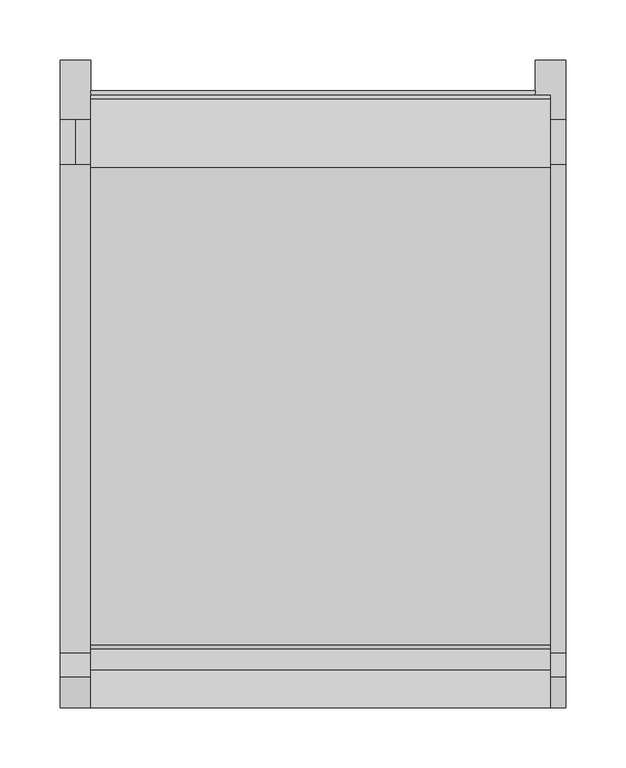
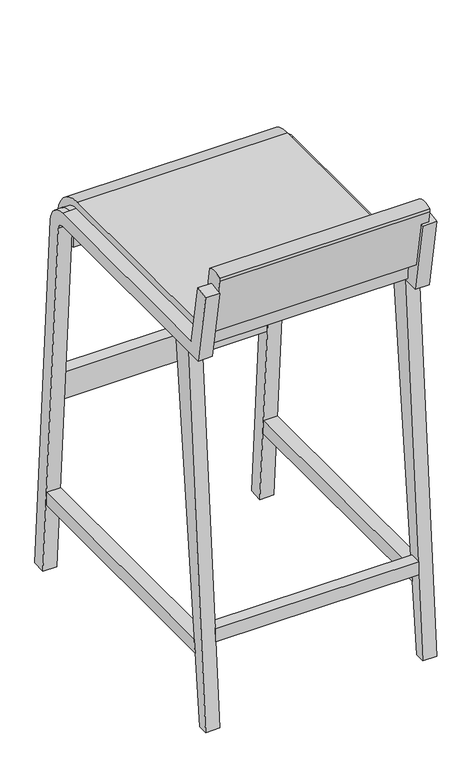
"""IFC4 building model written with IfcOpenShell, lengths in millimetres: furniture geometry, Bar_Stool_6722[1] : Bar_Stool_6722[1]."""

import ifcopenshell
import ifcopenshell.guid

model = None  # the IFC model being written
_history = None  # IfcOwnerHistory: only IFC2X3 demands one
_inside = {}  # id of a spatial element -> (the spatial element, [elements in it])
_under = {}  # id of a project, library or spatial element -> (it, [spatial elements below it])
_declared = {}  # id of a project -> (the project, [libraries it declares])
_typed = {}  # id of a type object -> (the type object, [elements of that type])
_made_of = {}  # id of a material, layer set ... -> (it, [elements and type objects made of it])


def new_model(schema):
    """Start an empty IFC model of exactly this schema.

    Asked for "IFC4X3", IfcOpenShell would pick the latest addendum, in which some entities
    have other attributes; the version numbers below select the first issue.
    IFC2X3 requires an IfcOwnerHistory on every rooted entity: one is made here for all.
    """
    global model, _history
    if schema == "IFC4X3":
        model = ifcopenshell.file(schema_version=(4, 3, 0, 0))
    else:
        model = ifcopenshell.file(schema=schema)
    _inside.clear()
    _under.clear()
    _declared.clear()
    _typed.clear()
    _made_of.clear()
    _history = None
    if model.schema == "IFC2X3":
        org = make("IfcOrganization", Name="unknown")
        user = make(
            "IfcPersonAndOrganization",
            ThePerson=make("IfcPerson", FamilyName="unknown"),
            TheOrganization=org,
        )
        app = make(
            "IfcApplication",
            ApplicationDeveloper=org,
            Version="unknown",
            ApplicationFullName="unknown",
            ApplicationIdentifier="unknown",
        )
        _history = make(
            "IfcOwnerHistory",
            OwningUser=user,
            OwningApplication=app,
            ChangeAction="ADDED",
            CreationDate=0,
        )
    return model


def make(cls, **values):
    """One entity of the class cls with the attributes given. An attribute that is None is left unset."""
    return model.create_entity(
        cls, **{name: value for name, value in values.items() if value is not None}
    )


def rooted(cls, **values):
    """An entity with a GlobalId (a new one), such as an element, a storey or a relation."""
    return make(cls, GlobalId=ifcopenshell.guid.new(), OwnerHistory=_history, **values)


def si_unit(unit_type, name, prefix=None):
    """IfcSIUnit, for example si_unit("LENGTHUNIT", "METRE", prefix="MILLI")."""
    return make("IfcSIUnit", UnitType=unit_type, Prefix=prefix, Name=name)


def assignment(units):
    """IfcUnitAssignment: the units of a project."""
    return None if units is None else make("IfcUnitAssignment", Units=units)


def point(xyz):
    """IfcCartesianPoint."""
    return None if xyz is None else make("IfcCartesianPoint", Coordinates=xyz)


def direction(xyz):
    """IfcDirection."""
    return None if xyz is None else make("IfcDirection", DirectionRatios=xyz)


def frame(location, z_axis=None, x_axis=None):
    """IfcAxis2Placement3D, a coordinate frame: its origin and axes. An axis left out is left unset."""
    return make(
        "IfcAxis2Placement3D",
        Location=point(location),
        Axis=direction(z_axis),
        RefDirection=direction(x_axis),
    )


def frame_2d(location, x_axis=None):
    """IfcAxis2Placement2D, a coordinate frame in the plane: its origin and x axis."""
    return make(
        "IfcAxis2Placement2D", Location=point(location), RefDirection=direction(x_axis)
    )


def origin():
    """The frame at (0, 0, 0) with its axes left unset."""
    return frame((0.0, 0.0, 0.0))


def place(relative_to, where):
    """IfcLocalPlacement: puts the frame where relative to a parent placement (None: the world)."""
    return make(
        "IfcLocalPlacement", PlacementRelTo=relative_to, RelativePlacement=where
    )


def context(
    kind, dimensions, precision=None, world=None, true_north=None, identifier=None
):
    """IfcGeometricRepresentationContext, for example the 3D "Model" context."""
    return make(
        "IfcGeometricRepresentationContext",
        ContextIdentifier=identifier,
        ContextType=kind,
        CoordinateSpaceDimension=dimensions,
        Precision=precision,
        WorldCoordinateSystem=world,
        TrueNorth=true_north,
    )


def project(units=None, contexts=None):
    """IfcProject with its units and contexts."""
    return rooted(
        "IfcProject",
        Name="project",
        RepresentationContexts=contexts,
        UnitsInContext=assignment(units),
    )


def spatial(cls, under=None, at=None, **own):
    """A site, building, storey or space (cls), placed at a placement, below another one or the project."""
    s = rooted(cls, ObjectPlacement=at, **own)
    if under is not None:
        _under.setdefault(under.id(), (under, []))[1].append(s)
    return s


def polyline(points):
    """IfcPolyline through the points."""
    return make("IfcPolyline", Points=[point(p) for p in points])


def circle_curve(where, radius):
    """IfcCircle in the frame where."""
    return make("IfcCircle", Position=where, Radius=radius)


def trimmed(basis, trim1, trim2, sense, master):
    """IfcTrimmedCurve: the piece of a basis curve between two trims."""
    return make(
        "IfcTrimmedCurve",
        BasisCurve=basis,
        Trim1=trim1,
        Trim2=trim2,
        SenseAgreement=sense,
        MasterRepresentation=master,
    )


def segment(curve, same_sense, transition):
    """IfcCompositeCurveSegment."""
    return make(
        "IfcCompositeCurveSegment",
        Transition=transition,
        SameSense=same_sense,
        ParentCurve=curve,
    )


def composite_curve(segments, self_intersect=None):
    """IfcCompositeCurve: segments joined end to end."""
    return make("IfcCompositeCurve", Segments=segments, SelfIntersect=self_intersect)


def outline(outer, holes=None, kind="AREA"):
    """IfcArbitraryClosedProfileDef: a profile drawn as a closed curve; with holes, ...WithVoids."""
    if holes is None:
        return make("IfcArbitraryClosedProfileDef", ProfileType=kind, OuterCurve=outer)
    return make(
        "IfcArbitraryProfileDefWithVoids",
        ProfileType=kind,
        OuterCurve=outer,
        InnerCurves=holes,
    )


def extrude(swept, where, along, depth):
    """IfcExtrudedAreaSolid: the profile swept, set in the frame where, extruded along a direction by depth."""
    return make(
        "IfcExtrudedAreaSolid",
        SweptArea=swept,
        Position=where,
        ExtrudedDirection=direction(along),
        Depth=depth,
    )


def shape(context_of_items, identifier, shape_type, items):
    """IfcShapeRepresentation: the items that make up one representation, for example the "Body"."""
    return make(
        "IfcShapeRepresentation",
        ContextOfItems=context_of_items,
        RepresentationIdentifier=identifier,
        RepresentationType=shape_type,
        Items=items,
    )


def source(mapping_origin, context_of_items, identifier, shape_type, items):
    """IfcRepresentationMap: a shape defined once, which mapped items show again and again."""
    return make(
        "IfcRepresentationMap",
        MappingOrigin=mapping_origin,
        MappedRepresentation=shape(context_of_items, identifier, shape_type, items),
    )


def transform(
    local_origin,
    x_axis=None,
    y_axis=None,
    z_axis=None,
    scale=None,
    scale2=None,
    scale3=None,
    uniform=True,
):
    """IfcCartesianTransformationOperator3D, or its non-uniform kind. x_axis, y_axis, z_axis: its Axis1, 2, 3."""
    if uniform:
        return make(
            "IfcCartesianTransformationOperator3D",
            Axis1=direction(x_axis),
            Axis2=direction(y_axis),
            LocalOrigin=point(local_origin),
            Scale=scale,
            Axis3=direction(z_axis),
        )
    return make(
        "IfcCartesianTransformationOperator3DnonUniform",
        Axis1=direction(x_axis),
        Axis2=direction(y_axis),
        LocalOrigin=point(local_origin),
        Scale=scale,
        Axis3=direction(z_axis),
        Scale2=scale2,
        Scale3=scale3,
    )


def mapped(mapping_source, mapping_target):
    """IfcMappedItem: shows the shape of a source again, moved by a transform."""
    return make(
        "IfcMappedItem", MappingSource=mapping_source, MappingTarget=mapping_target
    )


def made_of(thing, what):
    """Note that an element or type object is made of a material, layer set ...; save() writes the relation."""
    if what is not None:
        _made_of.setdefault(what.id(), (what, []))[1].append(thing)
    return thing


def element(
    cls,
    number,
    at=None,
    inside=None,
    cuts=None,
    type_object=None,
    material=None,
    context=None,
    identifier="Body",
    shape_type=None,
    held_by="IfcProductDefinitionShape",
    body=None,
    shapes=None,
    **own,
):
    """One element of the class cls, such as IfcWall. Its Tag is "e" and its number.

    at: its placement. inside: the storey or other place that contains it. cuts: it is an
    opening in that element (IfcRelVoidsElement). A single representation is given by context,
    identifier, shape_type and body (its items); several are given by shapes. held_by: the class
    of the entity that holds the representations. save() writes the other relations.
    """
    e = rooted(cls, Tag="e%d" % number, ObjectPlacement=at, **own)
    if body is not None:
        shapes = [shape(context, identifier, shape_type, body)]
    if shapes is not None:
        e.Representation = make(held_by, Representations=shapes)
    if inside is not None:
        _inside.setdefault(inside.id(), (inside, []))[1].append(e)
    if cuts is not None:
        rooted(
            "IfcRelVoidsElement", RelatingBuildingElement=cuts, RelatedOpeningElement=e
        )
    if type_object is not None:
        _typed.setdefault(type_object.id(), (type_object, []))[1].append(e)
    return made_of(e, material)


def aggregate(whole, parts):
    """IfcRelAggregates: a whole, such as a stair, and the parts it consists of."""
    return rooted("IfcRelAggregates", RelatingObject=whole, RelatedObjects=parts)


def save(model, path):
    """Write the relations noted so far, then the file.

    IfcRelAggregates (storeys below a building ...), IfcRelContainedInSpatialStructure (elements
    in a storey), IfcRelDefinesByType, IfcRelAssociatesMaterial and IfcRelDeclares: one each for
    every whole, place, type object, material and project.
    """
    for whole, parts in _under.values():
        aggregate(whole, parts)
    for where, things in _inside.values():
        rooted(
            "IfcRelContainedInSpatialStructure",
            RelatedElements=things,
            RelatingStructure=where,
        )
    for kind, things in _typed.values():
        rooted("IfcRelDefinesByType", RelatedObjects=things, RelatingType=kind)
    for what, things in _made_of.values():
        rooted("IfcRelAssociatesMaterial", RelatedObjects=things, RelatingMaterial=what)
    for by, libraries in _declared.values():
        rooted("IfcRelDeclares", RelatingContext=by, RelatedDefinitions=libraries)
    model.write(path)


def plane_surface(at):
    """IfcPlane: the flat surface through the origin of the frame at, square to its z axis."""
    return make("IfcPlane", Position=at)


def cylinder_surface(at, radius):
    """IfcCylindricalSurface: all points at the distance radius from the z axis of the frame at."""
    return make("IfcCylindricalSurface", Position=at, Radius=radius)


def revolved_surface(curve, axis_point, axis_direction):
    """IfcSurfaceOfRevolution: the curve turned about the line through axis_point along axis_direction."""
    return make(
        "IfcSurfaceOfRevolution",
        SweptCurve=make("IfcArbitraryOpenProfileDef", ProfileType="CURVE", Curve=curve),
        AxisPosition=make("IfcAxis1Placement", Location=point(axis_point), Axis=direction(axis_direction)),
    )


def advanced_brep(points, edges, surfaces, faces):
    """IfcAdvancedBrep: a solid bounded by faces that lie on surfaces and meet in shared edges.

    An edge is (start, end): straight between two places in points (the first is 0);
    or (start, end, curve); or (start, end, curve, False) where it runs against its curve.
    A face is (place in surfaces, loops), or (place, loops, False) where it looks against
    its surface's normal. A loop lists edges by number (the first is 1), with a minus sign
    where the edge is run from its end to its start. The first loop is the outer one.
    """
    corners = [point(p) for p in points]
    vertices = [make("IfcVertexPoint", VertexGeometry=c) for c in corners]
    made = []
    for start, end, *more in edges:
        made.append(
            make(
                "IfcEdgeCurve",
                EdgeStart=vertices[start],
                EdgeEnd=vertices[end],
                EdgeGeometry=more[0] if more else make("IfcPolyline", Points=[corners[start], corners[end]]),
                SameSense=more[1] if len(more) > 1 else True,
            )
        )
    hull = []
    for where, loops, *sense in faces:
        bounds = []
        for j, loop in enumerate(loops):
            ring = [make("IfcOrientedEdge", EdgeElement=made[abs(k) - 1], Orientation=k > 0) for k in loop]
            bounds.append(
                make(
                    "IfcFaceOuterBound" if j == 0 else "IfcFaceBound",
                    Bound=make("IfcEdgeLoop", EdgeList=ring),
                    Orientation=True,
                )
            )
        hull.append(make("IfcAdvancedFace", Bounds=bounds, FaceSurface=surfaces[where], SameSense=sense[0] if sense else True))
    return make("IfcAdvancedBrep", Outer=make("IfcClosedShell", CfsFaces=hull))


def furniture_48a66dd3(model_context):
    return source(origin(), model_context, "Body", "SolidModel", [
        advanced_brep(
        [(419.1, 25.0141169, 838.4759165), (393.7, 25.0141169, 838.4759165), (393.7, 0.0, 834.0652528), (419.1, 0.0, 834.0652528), (419.1, 45.2169423, 723.9), (393.7, 45.2169423, 723.9), (393.7, 450.0350637, 723.9), (393.7, 488.0397183, 688.4937383), (393.7, 536.7759384, 0.8979128), (393.7, 511.439502, -0.8979128), (393.7, 462.7032819, 686.6979128), (393.7, 450.0350637, 698.5), (393.7, 23.9038117, 698.5), (419.1, 23.9038117, 698.5), (419.1, 450.0350637, 698.5), (419.1, 462.7032819, 686.6979128), (419.1, 511.439502, -0.8979128), (419.1, 536.7759384, 0.8979128), (419.1, 488.0397183, 688.4937383), (419.1, 450.0350637, 723.9), (406.4, 450.0350637, 723.9), (406.4, 488.0397183, 688.4937383)],
        [
            (0, 1),
            (1, 2),
            (2, 3),
            (3, 0),
            (0, 4),
            (4, 5),
            (5, 1),
            (5, 6),
            (6, 7, circle_curve(frame((393.7, 450.0350637, 685.8), z_axis=(-1.0, 0.0, 0.0), x_axis=(0.0, 0.0, 1.0)), 38.1)),
            (7, 8),
            (8, 9),
            (9, 10),
            (10, 11, circle_curve(frame((393.7, 450.0350637, 685.8), z_axis=(1.0, 0.0, 0.0), x_axis=(0.0, 0.0, 1.0)), 12.7)),
            (11, 12),
            (12, 2),
            (12, 13),
            (13, 3),
            (13, 14),
            (14, 15, circle_curve(frame((419.1, 450.0350637, 685.8), z_axis=(-1.0, 0.0, 0.0), x_axis=(0.0, 0.0, 1.0)), 12.7)),
            (15, 16),
            (16, 17),
            (17, 18),
            (18, 19, circle_curve(frame((419.1, 450.0350637, 685.8), z_axis=(1.0, 0.0, 0.0), x_axis=(0.0, 0.0, 1.0)), 38.1)),
            (19, 4),
            (19, 20),
            (20, 6),
            (11, 14),
            (21, 20, circle_curve(frame((406.4, 450.0350637, 685.8), z_axis=(1.0, 0.0, 0.0), x_axis=(0.0, 0.0, 1.0)), 38.1)),
            (18, 21),
            (21, 7),
            (10, 15),
            (17, 8),
            (9, 16),
        ],
        [
            plane_surface(frame((406.4, 12.5070585, 836.2705846), z_axis=(0.0, -0.17364817766692853, 0.9848077530122085), x_axis=(1.0, 0.0, 0.0))),
            plane_surface(frame((406.4, 25.0141169, 838.4759165), z_axis=(0.0, 0.9848077530122085, 0.17364817766692814), x_axis=(0.0, 0.17364817766692814, -0.9848077530122085))),
            plane_surface(frame((393.7, 25.0141169, 838.4759165), z_axis=(-1.0, 0.0, 0.0), x_axis=(0.0, 0.17364817766692808, -0.9848077530122085))),
            plane_surface(frame((393.7, 0.0, 834.0652528), z_axis=(0.0, -0.9848077530122085, -0.17364817766692817), x_axis=(0.0, 0.17364817766692817, -0.9848077530122085))),
            plane_surface(frame((419.1, 0.0, 834.0652528), z_axis=(1.0000000000000002, 0.0, 0.0), x_axis=(0.0, 0.1736481776669284, -0.9848077530122085))),
            plane_surface(frame((406.4, 45.2169423, 723.9), z_axis=(0.0, 0.0, 1.0), x_axis=(0.0, 1.0, 0.0))),
            plane_surface(frame((393.7, 23.9038117, 698.5), z_axis=(0.0, 0.0, -1.0), x_axis=(0.0, 1.0, 0.0))),
            cylinder_surface(frame((406.4, 450.0350637, 685.8), z_axis=(-1.0, 0.0, 0.0), x_axis=(0.0, 0.0, 1.0)), 38.1),
            revolved_surface(polyline([(393.7, 450.0350637, 698.5), (419.1, 450.0350637, 698.5)]), (406.4, 450.0350637, 685.8), (-1.0, 0.0, 0.0)),
            plane_surface(frame((406.4, 488.0397183, 688.4937383), z_axis=(0.0, 0.9974974969901172, 0.07070179275273744), x_axis=(0.0, 0.07070179275273744, -0.9974974969901172))),
            plane_surface(frame((393.7, 462.7032819, 686.6979128), z_axis=(0.0, -0.9974974969901172, -0.07070179275273743), x_axis=(0.0, 0.07070179275273743, -0.9974974969901172))),
            plane_surface(frame((406.4, 524.1077202, 0.0), z_axis=(0.0, 0.07070179275273399, -0.9974974969901175), x_axis=(1.0, 0.0, 0.0))),
        ],
        [
            (0, [[1, 2, 3, 4]]),
            (1, [[5, 6, 7, -1]]),
            (2, [[-2, -7, 8, 9, 10, 11, 12, 13, 14, 15]]),
            (3, [[-3, -15, 16, 17]]),
            (4, [[-4, -17, 18, 19, 20, 21, 22, 23, 24, -5]]),
            (5, [[-6, -24, 25, 26, -8]]),
            (6, [[-16, -14, 27, -18]]),
            (7, [[28, -25, -23, 29]]),
            (7, [[-9, -26, -28, 30]]),
            (8, [[-19, -27, -13, 31]]),
            (9, [[-10, -30, -29, -22, 32]]),
            (10, [[-20, -31, -12, 33]]),
            (11, [[-32, -21, -33, -11]]),
        ],
    ),
        extrude(outline(composite_curve([segment(polyline([(48.4096386, 756.5644068), (44.0710693, 752.2258375), (19.1416957, 748.2774126), (0.0, 856.8353632), (0.0, 863.1853632)]), True, "CONTINUOUS"), segment(trimmed(circle_curve(frame_2d((15.7612691, 828.3540875)), 38.2313401), [point((0.0, 863.1853632))], [point((31.5225381, 863.1853632))], False, "CARTESIAN"), True, "CONTINUOUS"), segment(polyline([(31.5225381, 863.1853632), (48.4096386, 756.5644068)]), True, "CONTINUOUS")], self_intersect=False)), frame((25.4, 0.0, 0.0), z_axis=(1.0, 0.0, 0.0), x_axis=(0.0, 1.0, 0.0)), (0.0, 0.0, 1.0), 381.0),
        extrude(outline(composite_curve([segment(polyline([(51.6744261, 737.5144068), (447.8968201, 737.5144068)]), True, "CONTINUOUS"), segment(trimmed(circle_curve(frame_2d((447.8968201, 676.6245275)), 60.8898793), [point((447.8968201, 737.5144068))], [point((505.1145904, 697.4500928))], False, "CARTESIAN"), True, "CONTINUOUS"), segment(trimmed(circle_curve(frame_2d((460.5585493, 681.23302)), 47.4155486), [point((505.1145904, 697.4500928))], [point((484.2663236, 640.1699505))], False, "CARTESIAN"), True, "CONTINUOUS"), segment(polyline([(484.2663236, 640.1699505), (460.5585493, 643.13302), (460.5585493, 681.23302), (452.817441, 704.85), (46.417441, 704.85), (43.9498561, 733.0546243), (51.6744261, 737.5144068)]), True, "CONTINUOUS")], self_intersect=False)), frame((25.4, 0.0, 0.0), z_axis=(1.0, 0.0, 0.0), x_axis=(0.0, 1.0, 0.0)), (0.0, 0.0, 1.0), 381.0),
        extrude(outline(polyline([(393.7, 11.6871233), (25.4, 11.6871233), (25.4, 33.1441574), (393.7, 33.1441574), (393.7, 11.6871233)])), frame((0.0, 0.0, 157.9619127), z_axis=(0.0, 0.0, 1.0), x_axis=(1.0, 0.0, 0.0)), (0.0, 0.0, 1.0), 25.4),
        extrude(outline(polyline([(393.7, 488.2695397), (25.4, 488.2695397), (25.4, 511.439502), (393.7, 511.439502), (393.7, 488.2695397)])), frame((0.0, 0.0, 335.7619127), z_axis=(0.0, 0.0, 1.0), x_axis=(1.0, 0.0, 0.0)), (0.0, 0.0, 1.0), 50.8),
        extrude(outline(polyline([(500.1796497, 157.9619127), (500.1796497, 132.5619127), (32.9828185, 132.5619127), (35.652466, 157.9619127), (500.1796497, 157.9619127)])), frame((393.7, 0.0, 0.0), z_axis=(1.0, 0.0, 0.0), x_axis=(0.0, 1.0, 0.0)), (0.0, 0.0, 1.0), 25.4),
        extrude(outline(polyline([(500.1796497, 157.9619127), (500.1796497, 132.5619127), (32.9828185, 132.5619127), (35.652466, 157.9619127), (500.1796497, 157.9619127)])), frame((0.0, 0.0, 0.0), z_axis=(1.0, 0.0, 0.0), x_axis=(0.0, 1.0, 0.0)), (0.0, 0.0, 1.0), 25.4),
        extrude(outline(polyline([(0.0, 0.0), (55.3031462, 698.5), (92.4653083, 698.5), (19.05, 0.0), (0.0, 0.0)])), frame((393.7, 0.0, 0.0), z_axis=(1.0, 0.0, 0.0), x_axis=(0.0, 1.0, 0.0)), (0.0, 0.0, 1.0), 25.4),
        advanced_brep(
        [(25.4, 25.0141169, 838.4759165), (0.0, 25.0141169, 838.4759165), (0.0, 0.0, 834.0652528), (25.4, 0.0, 834.0652528), (25.4, 45.2169423, 723.9), (0.0, 45.2169423, 723.9), (0.0, 450.0350637, 723.9), (0.0, 488.0397183, 688.4937383), (0.0, 536.7759384, 0.8979128), (0.0, 511.439502, -0.8979128), (0.0, 462.7032819, 686.6979128), (0.0, 450.0350637, 698.5), (0.0, 23.9038117, 698.5), (25.4, 23.9038117, 698.5), (25.4, 450.0350637, 698.5), (25.4, 462.7032819, 686.6979128), (25.4, 511.439502, -0.8979128), (25.4, 536.7759384, 0.8979128), (25.4, 488.0397183, 688.4937383), (25.4, 450.0350637, 723.9), (12.7, 450.0350637, 723.9), (12.7, 488.0397183, 688.4937383)],
        [
            (0, 1),
            (1, 2),
            (2, 3),
            (3, 0),
            (0, 4),
            (4, 5),
            (5, 1),
            (5, 6),
            (6, 7, circle_curve(frame((0.0, 450.0350637, 685.8), z_axis=(-1.0, 0.0, 0.0), x_axis=(0.0, 0.0, 1.0)), 38.1)),
            (7, 8),
            (8, 9),
            (9, 10),
            (10, 11, circle_curve(frame((0.0, 450.0350637, 685.8), z_axis=(1.0, 0.0, 0.0), x_axis=(0.0, 0.0, 1.0)), 12.7)),
            (11, 12),
            (12, 2),
            (12, 13),
            (13, 3),
            (13, 14),
            (14, 15, circle_curve(frame((25.4, 450.0350637, 685.8), z_axis=(-1.0, 0.0, 0.0), x_axis=(0.0, 0.0, 1.0)), 12.7)),
            (15, 16),
            (16, 17),
            (17, 18),
            (18, 19, circle_curve(frame((25.4, 450.0350637, 685.8), z_axis=(1.0, 0.0, 0.0), x_axis=(0.0, 0.0, 1.0)), 38.1)),
            (19, 4),
            (19, 20),
            (20, 6),
            (11, 14),
            (21, 20, circle_curve(frame((12.7, 450.0350637, 685.8), z_axis=(1.0, 0.0, 0.0), x_axis=(0.0, 0.0, 1.0)), 38.1)),
            (18, 21),
            (21, 7),
            (10, 15),
            (17, 8),
            (9, 16),
        ],
        [
            plane_surface(frame((12.7, 12.5070585, 836.2705846), z_axis=(0.0, -0.17364817766692853, 0.9848077530122085), x_axis=(1.0, 0.0, 0.0))),
            plane_surface(frame((12.7, 25.0141169, 838.4759165), z_axis=(0.0, 0.9848077530122085, 0.173648177666928), x_axis=(0.0, 0.173648177666928, -0.9848077530122085))),
            plane_surface(frame((0.0, 25.0141169, 838.4759165), z_axis=(-1.0, 0.0, 0.0), x_axis=(0.0, 0.17364817766692875, -0.9848077530122084))),
            plane_surface(frame((0.0, 0.0, 834.0652528), z_axis=(0.0, -0.9848077530122084, -0.17364817766692883), x_axis=(0.0, 0.17364817766692883, -0.9848077530122084))),
            plane_surface(frame((25.4, 0.0, 834.0652528), z_axis=(1.0000000000000002, 0.0, 0.0), x_axis=(0.0, 0.1736481776669284, -0.9848077530122085))),
            plane_surface(frame((12.7, 45.2169423, 723.9), z_axis=(0.0, 0.0, 1.0), x_axis=(0.0, 1.0, 0.0))),
            plane_surface(frame((0.0, 23.9038117, 698.5), z_axis=(0.0, 0.0, -1.0), x_axis=(0.0, 1.0, 0.0))),
            cylinder_surface(frame((12.7, 450.0350637, 685.8), z_axis=(-1.0, 0.0, 0.0), x_axis=(0.0, 0.0, 1.0)), 38.1),
            revolved_surface(polyline([(0.0, 450.0350637, 698.5), (25.4, 450.0350637, 698.5)]), (12.7, 450.0350637, 685.8), (-1.0, 0.0, 0.0)),
            plane_surface(frame((12.7, 488.0397183, 688.4937383), z_axis=(0.0, 0.9974974969901172, 0.07070179275273744), x_axis=(0.0, 0.07070179275273744, -0.9974974969901172))),
            plane_surface(frame((0.0, 462.7032819, 686.6979128), z_axis=(0.0, -0.9974974969901172, -0.07070179275273743), x_axis=(0.0, 0.07070179275273743, -0.9974974969901172))),
            plane_surface(frame((12.7, 524.1077202, 0.0), z_axis=(0.0, 0.07070179275273399, -0.9974974969901175), x_axis=(1.0, 0.0, 0.0))),
        ],
        [
            (0, [[1, 2, 3, 4]]),
            (1, [[5, 6, 7, -1]]),
            (2, [[-2, -7, 8, 9, 10, 11, 12, 13, 14, 15]]),
            (3, [[-3, -15, 16, 17]]),
            (4, [[-4, -17, 18, 19, 20, 21, 22, 23, 24, -5]]),
            (5, [[-6, -24, 25, 26, -8]]),
            (6, [[-16, -14, 27, -18]]),
            (7, [[28, -25, -23, 29]]),
            (7, [[-9, -26, -28, 30]]),
            (8, [[-19, -27, -13, 31]]),
            (9, [[-10, -30, -29, -22, 32]]),
            (10, [[-20, -31, -12, 33]]),
            (11, [[-32, -21, -33, -11]]),
        ],
    ),
        extrude(outline(polyline([(0.0, 0.0), (55.3031462, 698.5), (92.4653083, 698.5), (19.05, 0.0), (0.0, 0.0)])), frame((0.0, 0.0, 0.0), z_axis=(1.0, 0.0, 0.0), x_axis=(0.0, 1.0, 0.0)), (0.0, 0.0, 1.0), 25.4),
    ])


if __name__ == "__main__":
    model = new_model("IFC4")
    model_context = context("Model", 3, world=origin())
    ifc_project = project(units=[si_unit("LENGTHUNIT", "METRE", prefix="MILLI")], contexts=[model_context])
    site = spatial("IfcSite", under=ifc_project)
    building = spatial("IfcBuilding", under=site)
    placement = place(None, origin())
    furniture_shape = furniture_48a66dd3(model_context)
    element("IfcFurniture", 1, ObjectType="Bar_Stool_6722[1] : Bar_Stool_6722[1]", at=placement, inside=building, context=model_context, shape_type="MappedRepresentation", body=[
        mapped(furniture_shape, transform((0.0, 0.0, 0.0), x_axis=(1.0, 0.0, 0.0), y_axis=(0.0, 1.0, 0.0), z_axis=(0.0, 0.0, 1.0))),
    ])
    save(model, "model.ifc")

# Revit data of these elements
# Type "Bar_Stool_6722[1] : Bar_Stool_6722[1]"
#   Seat = fab
#   Chair Legs = MET
# Element 1 (IfcFurniture, "Bar_Stool_6722[1] : Bar_Stool_6722[1]")
#   Materials on its faces: "MET", "fab"
# Materials
#   "fab": class "Leather", colour RGB 255 255 255, transparency 0, Cost = 0
#   "MET": class "Metal", colour RGB 189 187 185, transparency 0
